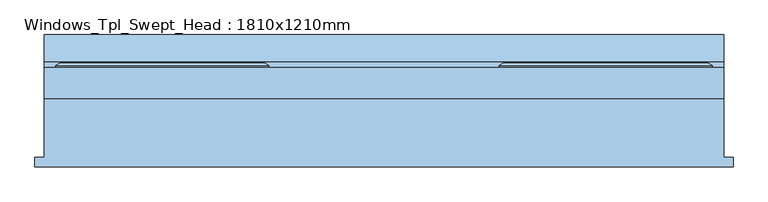
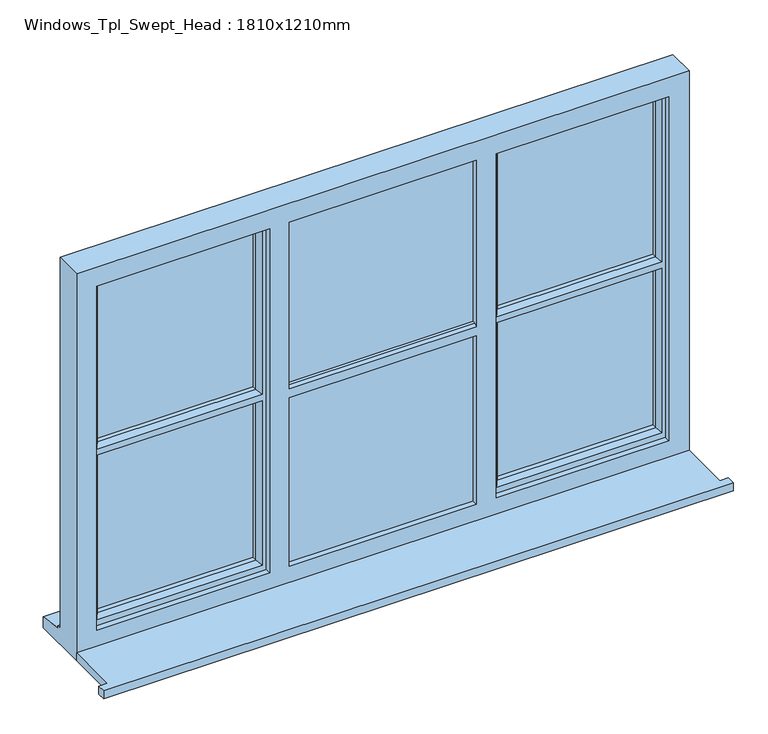
"""IFC4 building model written with IfcOpenShell, lengths in millimetres: window geometry, Windows_Tpl_Swept_Head : 1810x1210mm."""

from ifc_helpers import new_model, si_unit, point, frame, frame_2d, origin, place, context, project, spatial, polyline, circle_curve, trimmed, segment, composite_curve, outline, extrude, faceted_brep, source, transform, mapped, element, save


def windows_tpl_swept_head_1810x1210mm_ce76711b(model_context):
    return source(origin(), model_context, "Body", "SolidModel", [
        extrude(outline(polyline([(-1506.6666667, -161.5434322), (-1506.6666667, -136.5434322), (-1481.6666667, -136.5434322), (-1481.6666667, 20.4565678), (328.3333333, 20.4565678), (328.3333333, -136.5434322), (353.3333333, -136.5434322), (353.3333333, -161.5434322), (-1506.6666667, -161.5434322)])), frame((0.0, 0.0, 900.0), z_axis=(0.0, 0.0, 1.0), x_axis=(1.0, 0.0, 0.0)), (0.0, 0.0, 1.0), 25.0),
        extrude(outline(composite_curve([segment(polyline([(2050.0, -300.0), (2050.0, -853.3333333), (1968.0050976, -853.3333333)]), True, "CONTINUOUS"), segment(trimmed(circle_curve(frame_2d((1325.0, -576.6666667)), 700.0), [point((1968.0050976, -853.3333333))], [point((1968.0050976, -300.0))], True, "CARTESIAN"), True, "CONTINUOUS"), segment(polyline([(1968.0050976, -300.0), (2050.0, -300.0)]), True, "CONTINUOUS")], self_intersect=False)), frame((0.0, 62.4565678, 0.0), z_axis=(0.0, 1.0, 0.0), x_axis=(0.0, 0.0, 1.0)), (0.0, 0.0, 1.0), 25.0),
        extrude(outline(composite_curve([segment(polyline([(2030.0, -220.0), (1984.6711091, -220.0)]), True, "CONTINUOUS"), segment(trimmed(circle_curve(frame_2d((1325.0, 14.1666667)), 700.0), [point((1984.6711091, -220.0))], [point((1984.6711091, 248.3333333))], True, "CARTESIAN"), True, "CONTINUOUS"), segment(polyline([(1984.6711091, 248.3333333), (2030.0, 248.3333333), (2030.0, -220.0)]), True, "CONTINUOUS")], self_intersect=False)), frame((0.0, 79.4565678, 0.0), z_axis=(0.0, 1.0, 0.0), x_axis=(0.0, 0.0, 1.0)), (0.0, 0.0, 1.0), 24.0),
        extrude(outline(composite_curve([segment(polyline([(2030.0, -933.3333333), (2030.0, -1401.6666667), (1984.6711091, -1401.6666667)]), True, "CONTINUOUS"), segment(trimmed(circle_curve(frame_2d((1325.0, -1167.5)), 700.0), [point((1984.6711091, -1401.6666667))], [point((1984.6711091, -933.3333333))], True, "CARTESIAN"), True, "CONTINUOUS"), segment(polyline([(1984.6711091, -933.3333333), (2030.0, -933.3333333)]), True, "CONTINUOUS")], self_intersect=False)), frame((0.0, 79.4565678, 0.0), z_axis=(0.0, 1.0, 0.0), x_axis=(0.0, 0.0, 1.0)), (0.0, 0.0, 1.0), 24.0),
        faceted_brep([(-270.0, 103.4565678, 2080.0), (-270.0, 109.2300705, 2080.0), (-270.0, 109.2300705, 953.0), (-270.0, 103.4565678, 953.0), (-260.0, 38.4565678, 2070.0), (-260.0, 103.4565678, 2070.0), (-260.0, 103.4565678, 963.0), (-260.0, 38.4565678, 963.0), (-220.0, 52.9494677, 2030.0), (-230.1480377, 38.4565678, 2040.1480377), (-230.1480377, 38.4565678, 1526.3519623), (-220.0, 52.9494677, 1536.5), (-230.1480377, 38.4565678, 992.8519623), (-220.0, 52.9494677, 1003.0), (-220.0, 52.9494677, 1496.5), (-230.1480377, 38.4565678, 1506.6480377), (-220.0, 67.4565678, 2030.0), (-220.0, 67.4565678, 1536.5), (-220.0, 67.4565678, 1003.0), (-220.0, 67.4565678, 1496.5), (-230.0, 91.4565678, 1529.5), (-230.0, 91.4565678, 2040.0), (-230.0, 67.4565678, 2040.0), (-230.0, 67.4565678, 1529.5), (-230.0, 67.4565678, 1503.5), (-230.0, 67.4565678, 993.0), (-230.0, 91.4565678, 993.0), (-230.0, 91.4565678, 1503.5), (-220.0, 109.2300705, 2030.0), (-220.0, 91.4565678, 2030.0), (-220.0, 91.4565678, 1536.5), (-220.0, 109.2300705, 1536.5), (-220.0, 91.4565678, 1003.0), (-220.0, 109.2300705, 1003.0), (-220.0, 109.2300705, 1496.5), (-220.0, 91.4565678, 1496.5), (-237.4457548, 115.0035732, 2047.4457548), (-237.4457548, 115.0035732, 1519.0542452), (-237.4457548, 115.0035732, 985.5542452), (-237.4457548, 115.0035732, 1513.9457548), (-259.2153903, 115.0035732, 2069.2153903), (-259.2153903, 115.0035732, 963.7846097), (298.3333333, 109.2300705, 953.0), (298.3333333, 103.4565678, 953.0), (288.3333333, 103.4565678, 963.0), (288.3333333, 38.4565678, 963.0), (258.4813711, 38.4565678, 992.8519623), (248.3333333, 52.9494677, 1003.0), (248.3333333, 67.4565678, 1003.0), (258.3333333, 67.4565678, 993.0), (258.3333333, 91.4565678, 993.0), (248.3333333, 91.4565678, 1003.0), (248.3333333, 109.2300705, 1003.0), (265.7790881, 115.0035732, 985.5542452), (287.5487236, 115.0035732, 963.7846097), (298.3333333, 109.2300705, 2080.0), (298.3333333, 103.4565678, 2080.0), (288.3333333, 103.4565678, 2070.0), (288.3333333, 38.4565678, 2070.0), (258.4813711, 38.4565678, 1506.6480377), (248.3333333, 52.9494677, 1496.5), (258.4813711, 38.4565678, 2040.1480377), (248.3333333, 52.9494677, 2030.0), (248.3333333, 52.9494677, 1536.5), (258.4813711, 38.4565678, 1526.3519623), (248.3333333, 67.4565678, 1496.5), (248.3333333, 67.4565678, 2030.0), (248.3333333, 67.4565678, 1536.5), (258.3333333, 91.4565678, 1503.5), (258.3333333, 67.4565678, 1503.5), (258.3333333, 67.4565678, 1529.5), (258.3333333, 67.4565678, 2040.0), (258.3333333, 91.4565678, 2040.0), (258.3333333, 91.4565678, 1529.5), (248.3333333, 91.4565678, 1496.5), (248.3333333, 109.2300705, 1496.5), (248.3333333, 91.4565678, 2030.0), (248.3333333, 109.2300705, 2030.0), (248.3333333, 109.2300705, 1536.5), (248.3333333, 91.4565678, 1536.5), (265.7790881, 115.0035732, 1513.9457548), (265.7790881, 115.0035732, 2047.4457548), (265.7790881, 115.0035732, 1519.0542452), (287.5487236, 115.0035732, 2069.2153903)], [[[0, 1, 2, 3]], [[4, 5, 6, 7]], [[8, 9, 10, 11]], [[12, 13, 14, 15]], [[16, 8, 11, 17]], [[13, 18, 19, 14]], [[20, 21, 22, 23]], [[24, 25, 26, 27]], [[28, 29, 30, 31]], [[32, 33, 34, 35]], [[36, 28, 31, 37]], [[33, 38, 39, 34]], [[2, 1, 40, 41]], [[3, 2, 42, 43]], [[7, 6, 44, 45]], [[13, 12, 46, 47]], [[18, 13, 47, 48]], [[26, 25, 49, 50]], [[33, 32, 51, 52]], [[38, 33, 52, 53]], [[2, 41, 54, 42]], [[43, 42, 55, 56]], [[45, 44, 57, 58]], [[47, 46, 59, 60]], [[61, 62, 63, 64]], [[48, 47, 60, 65]], [[62, 66, 67, 63]], [[68, 50, 49, 69]], [[70, 71, 72, 73]], [[52, 51, 74, 75]], [[76, 77, 78, 79]], [[53, 52, 75, 80]], [[77, 81, 82, 78]], [[42, 54, 83, 55]], [[1, 0, 56, 55]], [[0, 3, 43, 56], [6, 5, 57, 44]], [[5, 4, 58, 57]], [[4, 7, 45, 58], [46, 12, 15, 59], [61, 64, 10, 9]], [[9, 8, 62, 61]], [[8, 16, 66, 62]], [[49, 25, 24, 69], [18, 48, 65, 19]], [[22, 71, 70, 23], [66, 16, 17, 67]], [[22, 21, 72, 71]], [[26, 50, 68, 27], [32, 35, 74, 51]], [[72, 21, 20, 73], [76, 79, 30, 29]], [[29, 28, 77, 76]], [[28, 36, 81, 77]], [[41, 40, 83, 54], [36, 37, 82, 81], [38, 53, 80, 39]], [[40, 1, 55, 83]], [[82, 37, 31, 78]], [[30, 79, 78, 31]], [[73, 20, 23, 70]], [[11, 63, 67, 17]], [[10, 64, 63, 11]], [[59, 15, 14, 60]], [[60, 14, 19, 65]], [[27, 68, 69, 24]], [[74, 35, 34, 75]], [[39, 80, 75, 34]]]),
        faceted_brep([(-883.3333333, 103.4565678, 2080.0), (-883.3333333, 109.2300705, 2080.0), (-1451.6666667, 109.2300705, 2080.0), (-1451.6666667, 103.4565678, 2080.0), (-893.3333333, 38.4565678, 2070.0), (-893.3333333, 103.4565678, 2070.0), (-1441.6666667, 103.4565678, 2070.0), (-1441.6666667, 38.4565678, 2070.0), (-933.3333333, 52.9494677, 2030.0), (-923.1852956, 38.4565678, 2040.1480377), (-1411.8147044, 38.4565678, 2040.1480377), (-1401.6666667, 52.9494677, 2030.0), (-1401.6666667, 67.4565678, 2030.0), (-933.3333333, 67.4565678, 2030.0), (-923.3333333, 91.4565678, 2040.0), (-923.3333333, 67.4565678, 2040.0), (-1411.6666667, 67.4565678, 2040.0), (-1411.6666667, 91.4565678, 2040.0), (-933.3333333, 109.2300705, 2030.0), (-933.3333333, 91.4565678, 2030.0), (-1401.6666667, 91.4565678, 2030.0), (-1401.6666667, 109.2300705, 2030.0), (-1419.1124215, 115.0035732, 2047.4457548), (-915.8875785, 115.0035732, 2047.4457548), (-894.117943, 115.0035732, 2069.2153903), (-1440.882057, 115.0035732, 2069.2153903), (-1451.6666667, 109.2300705, 953.0), (-1451.6666667, 103.4565678, 953.0), (-1441.6666667, 103.4565678, 963.0), (-1441.6666667, 38.4565678, 963.0), (-1411.8147044, 38.4565678, 1526.3519623), (-1401.6666667, 52.9494677, 1536.5), (-1411.8147044, 38.4565678, 992.8519623), (-1401.6666667, 52.9494677, 1003.0), (-1401.6666667, 52.9494677, 1496.5), (-1411.8147044, 38.4565678, 1506.6480377), (-1401.6666667, 67.4565678, 1536.5), (-1401.6666667, 67.4565678, 1003.0), (-1401.6666667, 67.4565678, 1496.5), (-1411.6666667, 91.4565678, 1529.5), (-1411.6666667, 67.4565678, 1529.5), (-1411.6666667, 67.4565678, 1503.5), (-1411.6666667, 67.4565678, 993.0), (-1411.6666667, 91.4565678, 993.0), (-1411.6666667, 91.4565678, 1503.5), (-1401.6666667, 91.4565678, 1536.5), (-1401.6666667, 109.2300705, 1536.5), (-1401.6666667, 91.4565678, 1003.0), (-1401.6666667, 109.2300705, 1003.0), (-1401.6666667, 109.2300705, 1496.5), (-1401.6666667, 91.4565678, 1496.5), (-1419.1124215, 115.0035732, 1519.0542452), (-1419.1124215, 115.0035732, 985.5542452), (-1419.1124215, 115.0035732, 1513.9457548), (-1440.882057, 115.0035732, 963.7846097), (-883.3333333, 109.2300705, 953.0), (-883.3333333, 103.4565678, 953.0), (-893.3333333, 103.4565678, 963.0), (-893.3333333, 38.4565678, 963.0), (-923.1852956, 38.4565678, 1526.3519623), (-923.1852956, 38.4565678, 1506.6480377), (-923.1852956, 38.4565678, 992.8519623), (-933.3333333, 52.9494677, 1003.0), (-933.3333333, 67.4565678, 1003.0), (-923.3333333, 67.4565678, 1529.5), (-933.3333333, 67.4565678, 1536.5), (-923.3333333, 67.4565678, 993.0), (-923.3333333, 67.4565678, 1503.5), (-933.3333333, 67.4565678, 1496.5), (-923.3333333, 91.4565678, 993.0), (-923.3333333, 91.4565678, 1529.5), (-933.3333333, 91.4565678, 1536.5), (-923.3333333, 91.4565678, 1503.5), (-933.3333333, 91.4565678, 1496.5), (-933.3333333, 91.4565678, 1003.0), (-933.3333333, 109.2300705, 1003.0), (-915.8875785, 115.0035732, 985.5542452), (-894.117943, 115.0035732, 963.7846097), (-915.8875785, 115.0035732, 1519.0542452), (-915.8875785, 115.0035732, 1513.9457548), (-933.3333333, 52.9494677, 1536.5), (-933.3333333, 52.9494677, 1496.5), (-933.3333333, 109.2300705, 1536.5), (-933.3333333, 109.2300705, 1496.5)], [[[0, 1, 2, 3]], [[4, 5, 6, 7]], [[8, 9, 10, 11]], [[8, 11, 12, 13]], [[14, 15, 16, 17]], [[18, 19, 20, 21]], [[18, 21, 22, 23]], [[2, 1, 24, 25]], [[3, 2, 26, 27]], [[7, 6, 28, 29]], [[11, 10, 30, 31]], [[32, 33, 34, 35]], [[12, 11, 31, 36]], [[33, 37, 38, 34]], [[39, 17, 16, 40]], [[41, 42, 43, 44]], [[21, 20, 45, 46]], [[47, 48, 49, 50]], [[22, 21, 46, 51]], [[48, 52, 53, 49]], [[2, 25, 54, 26]], [[27, 26, 55, 56]], [[0, 3, 27, 56], [6, 5, 57, 28]], [[29, 28, 57, 58]], [[4, 7, 29, 58], [10, 9, 59, 30], [32, 35, 60, 61]], [[33, 32, 61, 62]], [[37, 33, 62, 63]], [[16, 15, 64, 40], [13, 12, 36, 65]], [[66, 42, 41, 67], [37, 63, 68, 38]], [[43, 42, 66, 69]], [[14, 17, 39, 70], [19, 71, 45, 20]], [[43, 69, 72, 44], [47, 50, 73, 74]], [[48, 47, 74, 75]], [[52, 48, 75, 76]], [[25, 24, 77, 54], [23, 22, 51, 78], [76, 79, 53, 52]], [[26, 54, 77, 55]], [[1, 0, 56, 55]], [[5, 4, 58, 57]], [[9, 8, 80, 59]], [[62, 61, 60, 81]], [[8, 13, 65, 80]], [[63, 62, 81, 68]], [[64, 15, 14, 70]], [[72, 69, 66, 67]], [[19, 18, 82, 71]], [[75, 74, 73, 83]], [[18, 23, 78, 82]], [[76, 75, 83, 79]], [[24, 1, 55, 77]], [[78, 51, 46, 82]], [[45, 71, 82, 46]], [[40, 64, 70, 39]], [[65, 36, 31, 80]], [[30, 59, 80, 31]], [[60, 35, 34, 81]], [[38, 68, 81, 34]], [[67, 41, 44, 72]], [[73, 50, 49, 83]], [[53, 79, 83, 49]]]),
        extrude(outline(polyline([(258.4813711, 67.4565678), (-230.0, 67.4565678), (-230.0, 91.4565678), (258.4813711, 91.4565678), (258.4813711, 67.4565678)])), frame((0.0, 0.0, 993.0), z_axis=(0.0, 0.0, 1.0), x_axis=(1.0, 0.0, 0.0)), (0.0, 0.0, 1.0), 513.6480377),
        extrude(outline(polyline([(258.4813711, 67.4565678), (-230.0, 67.4565678), (-230.0, 91.4565678), (258.4813711, 91.4565678), (258.4813711, 67.4565678)])), frame((0.0, 0.0, 1526.3519623), z_axis=(0.0, 0.0, 1.0), x_axis=(1.0, 0.0, 0.0)), (0.0, 0.0, 1.0), 513.6480377),
        extrude(outline(polyline([(-863.3333333, 62.4565678), (-290.0, 62.4565678), (-290.0, 38.4565678), (-863.3333333, 38.4565678), (-863.3333333, 62.4565678)])), frame((0.0, 0.0, 963.0), z_axis=(0.0, 0.0, 1.0), x_axis=(1.0, 0.0, 0.0)), (0.0, 0.0, 1.0), 540.5),
        extrude(outline(polyline([(-863.3333333, 62.4565678), (-290.0, 62.4565678), (-290.0, 38.4565678), (-863.3333333, 38.4565678), (-863.3333333, 62.4565678)])), frame((0.0, 0.0, 1529.5), z_axis=(0.0, 0.0, 1.0), x_axis=(1.0, 0.0, 0.0)), (0.0, 0.0, 1.0), 540.5),
        extrude(outline(polyline([(-923.3333333, 67.4565678), (-1411.6666667, 67.4565678), (-1411.6666667, 91.4565678), (-923.3333333, 91.4565678), (-923.3333333, 67.4565678)])), frame((0.0, 0.0, 1526.3519623), z_axis=(0.0, 0.0, 1.0), x_axis=(1.0, 0.0, 0.0)), (0.0, 0.0, 1.0), 513.6480377),
        extrude(outline(polyline([(-923.3333333, 67.4565678), (-1411.6666667, 67.4565678), (-1411.6666667, 91.4565678), (-923.3333333, 91.4565678), (-923.3333333, 67.4565678)])), frame((0.0, 0.0, 993.0), z_axis=(0.0, 0.0, 1.0), x_axis=(1.0, 0.0, 0.0)), (0.0, 0.0, 1.0), 513.6480377),
        faceted_brep([(-853.3333333, 38.4565678, 2050.0), (-853.3333333, 20.4565678, 2050.0), (-853.3333333, 20.4565678, 1530.8390708), (-853.3333333, 28.5412125, 1536.5), (-853.3333333, 38.4565678, 1536.5), (-853.3333333, 20.4565678, 975.0), (-853.3333333, 38.4565678, 975.0), (-853.3333333, 38.4565678, 1496.5), (-853.3333333, 28.5412125, 1496.5), (-853.3333333, 20.4565678, 1502.1609292), (328.3333333, 20.4565678, 2110.0), (-1481.6666667, 20.4565678, 2110.0), (-1481.6666667, 20.4565678, 900.0), (328.3333333, 20.4565678, 900.0), (-1421.6666667, 20.4565678, 2050.0), (-911.3333333, 20.4565678, 2050.0), (-911.3333333, 20.4565678, 975.0), (-1421.6666667, 20.4565678, 975.0), (-242.0, 20.4565678, 2050.0), (268.3333333, 20.4565678, 2050.0), (268.3333333, 20.4565678, 975.0), (-242.0, 20.4565678, 975.0), (-300.0, 20.4565678, 2050.0), (-300.0, 20.4565678, 1530.8390708), (-300.0, 20.4565678, 975.0), (-300.0, 20.4565678, 1502.1609292), (-911.3333333, 38.4565678, 2050.0), (-911.3333333, 38.4565678, 975.0), (-1441.6666667, 38.4565678, 2070.0), (-893.3333333, 38.4565678, 2070.0), (-893.3333333, 38.4565678, 963.0), (-1441.6666667, 38.4565678, 963.0), (-1421.6666667, 38.4565678, 2050.0), (-1421.6666667, 38.4565678, 975.0), (-863.3333333, 38.4565678, 2070.0), (-290.0, 38.4565678, 2070.0), (-290.0, 38.4565678, 1529.5), (-853.3333333, 38.4565678, 1529.5), (-853.3333333, 38.4565678, 1503.5), (-290.0, 38.4565678, 1503.5), (-290.0, 38.4565678, 963.0), (-863.3333333, 38.4565678, 963.0), (-300.0, 38.4565678, 2050.0), (-300.0, 38.4565678, 1536.5), (-300.0, 38.4565678, 975.0), (-300.0, 38.4565678, 1496.5), (-260.0, 38.4565678, 2070.0), (288.3333333, 38.4565678, 2070.0), (288.3333333, 38.4565678, 963.0), (-260.0, 38.4565678, 963.0), (268.3333333, 38.4565678, 2050.0), (-242.0, 38.4565678, 2050.0), (-242.0, 38.4565678, 975.0), (268.3333333, 38.4565678, 975.0), (-893.3333333, 103.4565678, 2070.0), (-893.3333333, 103.4565678, 963.0), (-1481.6666667, 103.4565678, 2110.0), (328.3333333, 103.4565678, 2110.0), (328.3333333, 103.4565678, 951.0), (-1481.6666667, 103.4565678, 951.0), (-1441.6666667, 103.4565678, 2070.0), (-1441.6666667, 103.4565678, 963.0), (-853.3333333, 103.4565678, 2070.0), (-853.3333333, 103.4565678, 963.0), (-300.0, 103.4565678, 963.0), (-300.0, 103.4565678, 2070.0), (288.3333333, 103.4565678, 963.0), (288.3333333, 103.4565678, 2070.0), (-260.0, 103.4565678, 2070.0), (-260.0, 103.4565678, 963.0), (-853.3333333, 98.4565678, 2070.0), (-853.3333333, 98.4565678, 2050.0), (-853.3333333, 62.4565678, 2050.0), (-853.3333333, 62.4565678, 1536.5), (-853.3333333, 80.2300705, 1536.5), (-853.3333333, 86.0035732, 1519.0542452), (-853.3333333, 86.0035732, 1513.9457548), (-853.3333333, 80.2300705, 1496.5), (-853.3333333, 62.4565678, 1496.5), (-853.3333333, 62.4565678, 975.0), (-853.3333333, 98.4565678, 975.0), (-853.3333333, 98.4565678, 963.0), (-290.0, 62.4565678, 1503.5), (-853.3333333, 62.4565678, 1503.5), (-853.3333333, 62.4565678, 1529.5), (-290.0, 62.4565678, 1529.5), (-290.0, 62.4565678, 2070.0), (-863.3333333, 62.4565678, 2070.0), (-863.3333333, 62.4565678, 963.0), (-290.0, 62.4565678, 963.0), (-300.0, 62.4565678, 2050.0), (-300.0, 62.4565678, 1536.5), (-300.0, 62.4565678, 1496.5), (-300.0, 62.4565678, 975.0), (-1481.6666667, 118.4565678, 949.68767), (-1481.6666667, 118.4565678, 944.7449676), (-1481.6666667, 190.9565678, 933.8088847), (-1481.6666667, 190.9565678, 900.0), (-300.0, 98.4565678, 2070.0), (328.3333333, 190.9565678, 900.0), (328.3333333, 190.9565678, 933.8088847), (328.3333333, 118.4565678, 944.7449676), (328.3333333, 118.4565678, 949.68767), (-300.0, 98.4565678, 963.0), (-300.0, 98.4565678, 975.0), (-300.0, 80.2300705, 1496.5), (-300.0, 86.0035732, 1513.9457548), (-300.0, 86.0035732, 1519.0542452), (-300.0, 80.2300705, 1536.5), (-300.0, 98.4565678, 2050.0), (-300.0, 28.5412125, 1536.5), (-300.0, 28.5412125, 1496.5)], [[[0, 1, 2, 3, 4]], [[5, 6, 7, 8, 9]], [[10, 11, 12, 13], [14, 15, 16, 17], [18, 19, 20, 21], [1, 22, 23, 2], [24, 5, 9, 25]], [[15, 26, 27, 16]], [[28, 29, 30, 31], [26, 32, 33, 27]], [[34, 35, 36, 37, 38, 39, 40, 41], [42, 0, 4, 43], [6, 44, 45, 7]], [[46, 47, 48, 49], [50, 51, 52, 53]], [[54, 55, 30, 29]], [[56, 57, 58, 59], [55, 54, 60, 61], [62, 63, 64, 65], [66, 67, 68, 69]], [[63, 62, 70, 71, 72, 73, 74, 75, 76, 77, 78, 79, 80, 81]], [[82, 83, 84, 85, 86, 87, 88, 89], [73, 72, 90, 91], [92, 93, 79, 78]], [[88, 87, 34, 41]], [[11, 56, 59, 94, 95, 96, 97, 12]], [[61, 60, 28, 31]], [[32, 14, 17, 33]], [[11, 10, 57, 56]], [[62, 65, 98, 70]], [[87, 86, 35, 34]], [[28, 60, 54, 29]], [[67, 47, 46, 68]], [[1, 0, 42, 22]], [[14, 32, 26, 15]], [[50, 19, 18, 51]], [[57, 10, 13, 99, 100, 101, 102, 58]], [[67, 66, 48, 47]], [[19, 50, 53, 20]], [[82, 89, 40, 39]], [[35, 86, 85, 36]], [[65, 64, 103, 104, 93, 92, 105, 106, 107, 108, 91, 90, 109, 98]], [[69, 68, 46, 49]], [[51, 18, 21, 52]], [[22, 42, 43, 110, 23]], [[44, 24, 25, 111, 45]], [[99, 13, 12, 97]], [[100, 99, 97, 96]], [[101, 100, 96, 95]], [[102, 101, 95, 94]], [[58, 102, 94, 59]], [[55, 61, 31, 30]], [[64, 63, 81, 103]], [[66, 69, 49, 48]], [[89, 88, 41, 40]], [[17, 16, 27, 33]], [[21, 20, 53, 52]], [[44, 6, 5, 24]], [[83, 38, 37, 84]], [[75, 107, 106, 76]], [[76, 106, 105, 77]], [[92, 78, 77, 105]], [[38, 83, 82, 39]], [[7, 45, 111, 8]], [[25, 9, 8, 111]], [[2, 23, 110, 3]], [[43, 4, 3, 110]], [[84, 37, 36, 85]], [[73, 91, 108, 74]], [[107, 75, 74, 108]], [[79, 93, 104, 80]], [[80, 104, 103, 81]], [[109, 71, 70, 98]], [[90, 72, 71, 109]]]),
    ])


if __name__ == "__main__":
    model = new_model("IFC4")
    model_context = context("Model", 3, world=origin())
    ifc_project = project(units=[si_unit("LENGTHUNIT", "METRE", prefix="MILLI")], contexts=[model_context])
    site = spatial("IfcSite", under=ifc_project)
    building = spatial("IfcBuilding", under=site)
    placement = place(None, origin())
    windows_tpl_swept_head_1810x1210mm_shape = windows_tpl_swept_head_1810x1210mm_ce76711b(model_context)
    element("IfcWindow", 1, ObjectType="Windows_Tpl_Swept_Head : 1810x1210mm", at=placement, inside=building, context=model_context, shape_type="MappedRepresentation", body=[
        mapped(windows_tpl_swept_head_1810x1210mm_shape, transform((0.0, 0.0, 0.0), x_axis=(1.0, 0.0, 0.0), y_axis=(0.0, 1.0, 0.0), z_axis=(0.0, 0.0, 1.0))),
    ])
    save(model, "model.ifc")

# Revit data of these elements
# Type "Windows_Tpl_Swept_Head : 1810x1210mm"
#   Type Mark = "55"
#   Operation = "TriplePanelVertical"
#   Construction Type Id = "GSP4R"
#   Manufacturer = "Revit"
#   Keynote = "L10"
#   Analytic Construction = "1/8 in Pilkington single glazing"
#   Wrap Layers (Ext) from Ext = 102.5 mm
#   Wrap Layers (Int) from Ext = 177.5 mm
#   Window Board Projection = 25 mm
#   Window Board Extension = 25 mm
#   Visual Light Transmittance = 0.9
#   Solar Heat Gain Coefficient = 0.78
#   Rough Width = 1810 mm
#   Rough Height = 1210 mm
#   Radius - Swept Head = 700 mm
#   Height = 1210 mm
#   Width = 1810 mm
#   Heat Transfer Coefficient (U) = 3.6886 W/(m²·K)
#   Glazing Thickness = 24 mm
#   FrameOffset - External = 50 mm
#   Frame Depth = 65 mm
#   Default Head Height = 2110 mm
#   Cill Depth = 87.5 mm
#   Cavity Closer Width = 50 mm
#   Cavity Closer Offset from Ext = 102.5 mm
#   Cavity Closer Depth = 85 mm
#   Vis - Cavity Closers = yes
#   Material Trim = Window Frame
#   Material Glass = Glass
#   Material Frame = Window Frame
#   Wall Closure = (empty or 0)
# Element 1 (IfcWindow, "Windows_Tpl_Swept_Head : 1810x1210mm")
#   Materials on its faces: "Window Frame", "Glass"
# Materials
#   "Window Frame": class "Miscellaneous", colour RGB 249 249 249, transparency 0, Keynote = "L10", Cost = 0
#   "Glass": class "Glass", colour RGB 0 128 192, transparency 0.9, Description = "Soda Lime Glass", Cost = 0
